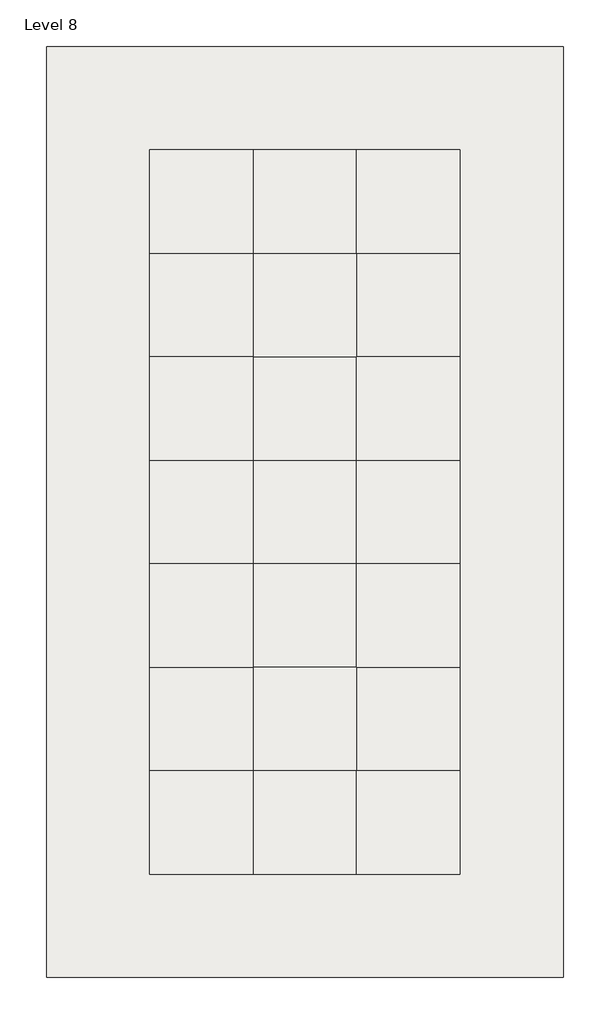
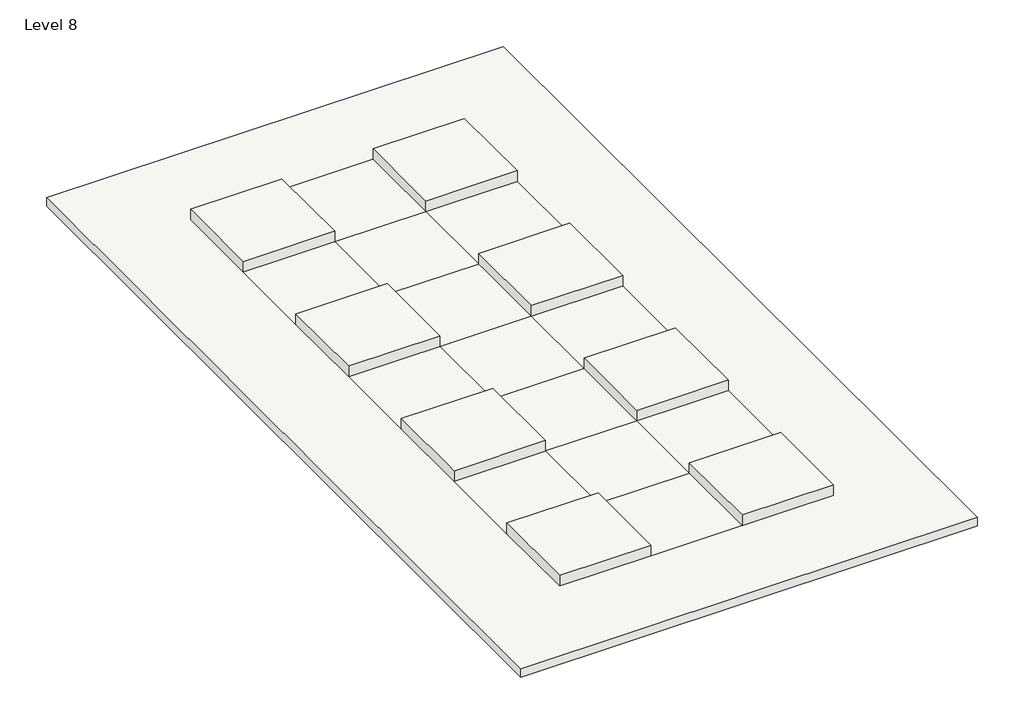
# One storey: 9 roofs.
"""IFC4 building model written with IfcOpenShell, lengths in millimetres."""

import ifcopenshell
import ifcopenshell.guid

model = None  # the IFC model being written
_history = None  # IfcOwnerHistory: only IFC2X3 demands one
_inside = {}  # id of a spatial element -> (the spatial element, [elements in it])
_under = {}  # id of a project, library or spatial element -> (it, [spatial elements below it])
_declared = {}  # id of a project -> (the project, [libraries it declares])
_typed = {}  # id of a type object -> (the type object, [elements of that type])
_made_of = {}  # id of a material, layer set ... -> (it, [elements and type objects made of it])


def new_model(schema):
    """Start an empty IFC model of exactly this schema.

    Asked for "IFC4X3", IfcOpenShell would pick the latest addendum, in which some entities
    have other attributes; the version numbers below select the first issue.
    IFC2X3 requires an IfcOwnerHistory on every rooted entity: one is made here for all.
    """
    global model, _history
    if schema == "IFC4X3":
        model = ifcopenshell.file(schema_version=(4, 3, 0, 0))
    else:
        model = ifcopenshell.file(schema=schema)
    _inside.clear()
    _under.clear()
    _declared.clear()
    _typed.clear()
    _made_of.clear()
    _history = None
    if model.schema == "IFC2X3":
        org = make("IfcOrganization", Name="unknown")
        user = make(
            "IfcPersonAndOrganization",
            ThePerson=make("IfcPerson", FamilyName="unknown"),
            TheOrganization=org,
        )
        app = make(
            "IfcApplication",
            ApplicationDeveloper=org,
            Version="unknown",
            ApplicationFullName="unknown",
            ApplicationIdentifier="unknown",
        )
        _history = make(
            "IfcOwnerHistory",
            OwningUser=user,
            OwningApplication=app,
            ChangeAction="ADDED",
            CreationDate=0,
        )
    return model


def make(cls, **values):
    """One entity of the class cls with the attributes given. An attribute that is None is left unset."""
    return model.create_entity(
        cls, **{name: value for name, value in values.items() if value is not None}
    )


def rooted(cls, **values):
    """An entity with a GlobalId (a new one), such as an element, a storey or a relation."""
    return make(cls, GlobalId=ifcopenshell.guid.new(), OwnerHistory=_history, **values)


def si_unit(unit_type, name, prefix=None):
    """IfcSIUnit, for example si_unit("LENGTHUNIT", "METRE", prefix="MILLI")."""
    return make("IfcSIUnit", UnitType=unit_type, Prefix=prefix, Name=name)


def assignment(units):
    """IfcUnitAssignment: the units of a project."""
    return None if units is None else make("IfcUnitAssignment", Units=units)


def point(xyz):
    """IfcCartesianPoint."""
    return None if xyz is None else make("IfcCartesianPoint", Coordinates=xyz)


def direction(xyz):
    """IfcDirection."""
    return None if xyz is None else make("IfcDirection", DirectionRatios=xyz)


def frame(location, z_axis=None, x_axis=None):
    """IfcAxis2Placement3D, a coordinate frame: its origin and axes. An axis left out is left unset."""
    return make(
        "IfcAxis2Placement3D",
        Location=point(location),
        Axis=direction(z_axis),
        RefDirection=direction(x_axis),
    )


def origin():
    """The frame at (0, 0, 0) with its axes left unset."""
    return frame((0.0, 0.0, 0.0))


def place(relative_to, where):
    """IfcLocalPlacement: puts the frame where relative to a parent placement (None: the world)."""
    return make(
        "IfcLocalPlacement", PlacementRelTo=relative_to, RelativePlacement=where
    )


def context(
    kind, dimensions, precision=None, world=None, true_north=None, identifier=None
):
    """IfcGeometricRepresentationContext, for example the 3D "Model" context."""
    return make(
        "IfcGeometricRepresentationContext",
        ContextIdentifier=identifier,
        ContextType=kind,
        CoordinateSpaceDimension=dimensions,
        Precision=precision,
        WorldCoordinateSystem=world,
        TrueNorth=true_north,
    )


def project(units=None, contexts=None):
    """IfcProject with its units and contexts."""
    return rooted(
        "IfcProject",
        Name="project",
        RepresentationContexts=contexts,
        UnitsInContext=assignment(units),
    )


def spatial(cls, under=None, at=None, **own):
    """A site, building, storey or space (cls), placed at a placement, below another one or the project."""
    s = rooted(cls, ObjectPlacement=at, **own)
    if under is not None:
        _under.setdefault(under.id(), (under, []))[1].append(s)
    return s


def faces_of(points, faces, orient=None, outer=None):
    """IfcFace entities. A face is a list of loops; a loop is a list of indices into points, from 0.

    orient and outer hold one flag for each loop. By default every Orientation is true, the
    first loop of a face is its IfcFaceOuterBound and the others are IfcFaceBound.
    """
    made = []
    for i, loops in enumerate(faces):
        bounds = []
        for j, loop in enumerate(loops):
            is_outer = j == 0 if outer is None else outer[i][j]
            bounds.append(
                make(
                    "IfcFaceOuterBound" if is_outer else "IfcFaceBound",
                    Bound=make("IfcPolyLoop", Polygon=[points[k] for k in loop]),
                    Orientation=True if orient is None else orient[i][j],
                )
            )
        made.append(make("IfcFace", Bounds=bounds))
    return made


def faceted_brep(points, faces, orient=None, outer=None, voids=None):
    """IfcFacetedBrep: a solid bounded by flat faces; with voids (closed shells), ...WithVoids."""
    shared = [point(p) for p in points]
    hull = make("IfcClosedShell", CfsFaces=faces_of(shared, faces, orient, outer))
    if voids is None:
        return make("IfcFacetedBrep", Outer=hull)
    return make(
        "IfcFacetedBrepWithVoids",
        Outer=hull,
        Voids=[
            make(cls, CfsFaces=faces_of(shared, fs, o, b)) for cls, fs, o, b in voids
        ],
    )


def shape(context_of_items, identifier, shape_type, items):
    """IfcShapeRepresentation: the items that make up one representation, for example the "Body"."""
    return make(
        "IfcShapeRepresentation",
        ContextOfItems=context_of_items,
        RepresentationIdentifier=identifier,
        RepresentationType=shape_type,
        Items=items,
    )


def made_of(thing, what):
    """Note that an element or type object is made of a material, layer set ...; save() writes the relation."""
    if what is not None:
        _made_of.setdefault(what.id(), (what, []))[1].append(thing)
    return thing


def element(
    cls,
    number,
    at=None,
    inside=None,
    cuts=None,
    type_object=None,
    material=None,
    context=None,
    identifier="Body",
    shape_type=None,
    held_by="IfcProductDefinitionShape",
    body=None,
    shapes=None,
    **own,
):
    """One element of the class cls, such as IfcWall. Its Tag is "e" and its number.

    at: its placement. inside: the storey or other place that contains it. cuts: it is an
    opening in that element (IfcRelVoidsElement). A single representation is given by context,
    identifier, shape_type and body (its items); several are given by shapes. held_by: the class
    of the entity that holds the representations. save() writes the other relations.
    """
    e = rooted(cls, Tag="e%d" % number, ObjectPlacement=at, **own)
    if body is not None:
        shapes = [shape(context, identifier, shape_type, body)]
    if shapes is not None:
        e.Representation = make(held_by, Representations=shapes)
    if inside is not None:
        _inside.setdefault(inside.id(), (inside, []))[1].append(e)
    if cuts is not None:
        rooted(
            "IfcRelVoidsElement", RelatingBuildingElement=cuts, RelatedOpeningElement=e
        )
    if type_object is not None:
        _typed.setdefault(type_object.id(), (type_object, []))[1].append(e)
    return made_of(e, material)


def aggregate(whole, parts):
    """IfcRelAggregates: a whole, such as a stair, and the parts it consists of."""
    return rooted("IfcRelAggregates", RelatingObject=whole, RelatedObjects=parts)


def save(model, path):
    """Write the relations noted so far, then the file.

    IfcRelAggregates (storeys below a building ...), IfcRelContainedInSpatialStructure (elements
    in a storey), IfcRelDefinesByType, IfcRelAssociatesMaterial and IfcRelDeclares: one each for
    every whole, place, type object, material and project.
    """
    for whole, parts in _under.values():
        aggregate(whole, parts)
    for where, things in _inside.values():
        rooted(
            "IfcRelContainedInSpatialStructure",
            RelatedElements=things,
            RelatingStructure=where,
        )
    for kind, things in _typed.values():
        rooted("IfcRelDefinesByType", RelatedObjects=things, RelatingType=kind)
    for what, things in _made_of.values():
        rooted("IfcRelAssociatesMaterial", RelatedObjects=things, RelatingMaterial=what)
    for by, libraries in _declared.values():
        rooted("IfcRelDeclares", RelatingContext=by, RelatedDefinitions=libraries)
    model.write(path)


model = new_model("IFC4")

# Units and contexts
model_context = context("Model", 3, world=origin())
ifc_project = project(units=[si_unit("LENGTHUNIT", "METRE", prefix="MILLI")], contexts=[model_context])

# Site, building, storey
site = spatial("IfcSite", under=ifc_project)
building = spatial("IfcBuilding", under=site)
storey = spatial("IfcBuildingStorey", under=building, Name="Level 8", Elevation=32000.0)

# Roofs
placement = place(None, origin())
element("IfcRoof", 1, ObjectType="Bauder_RoofCoveringSystem_ExtensiveGreenRoofSystem_WildflowerBlanket", at=placement, inside=storey, context=model_context, shape_type="Brep", body=[
    faceted_brep([(-674.7340554, 1676.2074539, 32000.0), (1325.2659446, 1676.2074539, 32000.0), (1325.2659446, -323.7925461, 32000.0), (-674.7340554, -323.7925461, 32000.0), (1325.2659446, 1676.2074539, 32445.0), (-674.7340554, 1676.2074539, 32445.0), (-674.7340554, -323.7925461, 32445.0), (1325.2659446, -323.7925461, 32445.0), (1325.2659446, 1676.2074539, 32200.0), (-674.7340554, 1676.2074539, 32200.0), (-674.7340554, -323.7925461, 32200.0), (1325.2659446, -323.7925461, 32200.0)], [[[0, 1, 2, 3]], [[4, 5, 6, 7]], [[5, 4, 8, 1, 0, 9]], [[6, 5, 9, 0, 3, 10]], [[7, 6, 10, 3, 2, 11]], [[4, 7, 11, 2, 1, 8]]]),
])
element("IfcRoof", 2, ObjectType="Bauder_RoofCoveringSystem_ExtensiveGreenRoofSystem_WildflowerBlanket", at=placement, inside=storey, context=model_context, shape_type="Brep", body=[
    faceted_brep([(3325.2659446, 1676.2074539, 32000.0), (5325.2659446, 1676.2074539, 32000.0), (5325.2659446, -323.7925461, 32000.0), (3325.2659446, -323.7925461, 32000.0), (5325.2659446, 1676.2074539, 32445.0), (3325.2659446, 1676.2074539, 32445.0), (3325.2659446, -323.7925461, 32445.0), (5325.2659446, -323.7925461, 32445.0), (5325.2659446, 1676.2074539, 32200.0), (3325.2659446, 1676.2074539, 32200.0), (3325.2659446, -323.7925461, 32200.0), (5325.2659446, -323.7925461, 32200.0)], [[[0, 1, 2, 3]], [[4, 5, 6, 7]], [[5, 4, 8, 1, 0, 9]], [[6, 5, 9, 0, 3, 10]], [[7, 6, 10, 3, 2, 11]], [[4, 7, 11, 2, 1, 8]]]),
])
element("IfcRoof", 3, ObjectType="Bauder_RoofCoveringSystem_ExtensiveGreenRoofSystem_WildflowerBlanket", at=placement, inside=storey, context=model_context, shape_type="Brep", body=[
    faceted_brep([(3325.2659446, -2323.7925461, 32000.0), (5325.2659446, -2323.7925461, 32000.0), (5325.2659446, -4323.7925461, 32000.0), (3325.2659446, -4323.7925461, 32000.0), (5325.2659446, -2323.7925461, 32445.0), (3325.2659446, -2323.7925461, 32445.0), (3325.2659446, -4323.7925461, 32445.0), (5325.2659446, -4323.7925461, 32445.0), (5325.2659446, -2323.7925461, 32200.0), (3325.2659446, -2323.7925461, 32200.0), (3325.2659446, -4323.7925461, 32200.0), (5325.2659446, -4323.7925461, 32200.0)], [[[0, 1, 2, 3]], [[4, 5, 6, 7]], [[5, 4, 8, 1, 0, 9]], [[6, 5, 9, 0, 3, 10]], [[7, 6, 10, 3, 2, 11]], [[4, 7, 11, 2, 1, 8]]]),
])
element("IfcRoof", 4, ObjectType="Bauder_RoofCoveringSystem_ExtensiveGreenRoofSystem_WildflowerBlanket", at=placement, inside=storey, context=model_context, shape_type="Brep", body=[
    faceted_brep([(3325.2659446, -6323.7925461, 32000.0), (5325.2659446, -6323.7925461, 32000.0), (5325.2659446, -8323.7925461, 32000.0), (3325.2659446, -8323.7925461, 32000.0), (5325.2659446, -6323.7925461, 32445.0), (3325.2659446, -6323.7925461, 32445.0), (3325.2659446, -8323.7925461, 32445.0), (5325.2659446, -8323.7925461, 32445.0), (3325.2659446, -6323.7925461, 32200.0), (5325.2659446, -6323.7925461, 32200.0), (3325.2659446, -8323.7925461, 32200.0), (5325.2659446, -8323.7925461, 32200.0)], [[[0, 1, 2, 3]], [[4, 5, 6, 7]], [[0, 8, 5, 4, 9, 1]], [[3, 10, 6, 5, 8, 0]], [[2, 11, 7, 6, 10, 3]], [[1, 9, 4, 7, 11, 2]]]),
])
element("IfcRoof", 5, ObjectType="Bauder_RoofCoveringSystem_ExtensiveGreenRoofSystem_WildflowerBlanket", at=placement, inside=storey, context=model_context, shape_type="Brep", body=[
    faceted_brep([(3325.2659446, -10323.7925461, 32000.0), (5325.2659446, -10323.7925461, 32000.0), (5325.2659446, -12323.7925461, 32000.0), (3325.2659446, -12323.7925461, 32000.0), (5325.2659446, -10323.7925461, 32445.0), (3325.2659446, -10323.7925461, 32445.0), (3325.2659446, -12323.7925461, 32445.0), (5325.2659446, -12323.7925461, 32445.0), (3325.2659446, -10323.7925461, 32200.0), (5325.2659446, -10323.7925461, 32200.0), (3325.2659446, -12323.7925461, 32200.0), (5325.2659446, -12323.7925461, 32200.0)], [[[0, 1, 2, 3]], [[4, 5, 6, 7]], [[0, 8, 5, 4, 9, 1]], [[3, 10, 6, 5, 8, 0]], [[2, 11, 7, 6, 10, 3]], [[1, 9, 4, 7, 11, 2]]]),
])
element("IfcRoof", 6, ObjectType="Bauder_RoofCoveringSystem_ExtensiveGreenRoofSystem_WildflowerBlanket", at=placement, inside=storey, context=model_context, shape_type="Brep", body=[
    faceted_brep([(-674.7340554, -10323.7925461, 32000.0), (1325.2659446, -10323.7925461, 32000.0), (1325.2659446, -12323.7925461, 32000.0), (-674.7340554, -12323.7925461, 32000.0), (1325.2659446, -10323.7925461, 32445.0), (-674.7340554, -10323.7925461, 32445.0), (-674.7340554, -12323.7925461, 32445.0), (1325.2659446, -12323.7925461, 32445.0), (1325.2659446, -10323.7925461, 32200.0), (-674.7340554, -10323.7925461, 32200.0), (-674.7340554, -12323.7925461, 32200.0), (1325.2659446, -12323.7925461, 32200.0)], [[[0, 1, 2, 3]], [[4, 5, 6, 7]], [[5, 4, 8, 1, 0, 9]], [[6, 5, 9, 0, 3, 10]], [[7, 6, 10, 3, 2, 11]], [[4, 7, 11, 2, 1, 8]]]),
])
element("IfcRoof", 7, ObjectType="Bauder_RoofCoveringSystem_ExtensiveGreenRoofSystem_WildflowerBlanket", at=placement, inside=storey, context=model_context, shape_type="Brep", body=[
    faceted_brep([(-674.7340554, -6323.7925461, 32000.0), (1325.2659446, -6323.7925461, 32000.0), (1325.2659446, -8323.7925461, 32000.0), (-674.7340554, -8323.7925461, 32000.0), (1325.2659446, -6323.7925461, 32445.0), (-674.7340554, -6323.7925461, 32445.0), (-674.7340554, -8323.7925461, 32445.0), (1325.2659446, -8323.7925461, 32445.0), (1325.2659446, -6323.7925461, 32200.0), (-674.7340554, -6323.7925461, 32200.0), (-674.7340554, -8323.7925461, 32200.0), (1325.2659446, -8323.7925461, 32200.0)], [[[0, 1, 2, 3]], [[4, 5, 6, 7]], [[5, 4, 8, 1, 0, 9]], [[6, 5, 9, 0, 3, 10]], [[7, 6, 10, 3, 2, 11]], [[4, 7, 11, 2, 1, 8]]]),
])
element("IfcRoof", 8, ObjectType="Bauder_RoofCoveringSystem_ExtensiveGreenRoofSystem_WildflowerBlanket", at=placement, inside=storey, context=model_context, shape_type="Brep", body=[
    faceted_brep([(-674.7340554, -2323.7925461, 32000.0), (1325.2659446, -2323.7925461, 32000.0), (1325.2659446, -4323.7925461, 32000.0), (-674.7340554, -4323.7925461, 32000.0), (1325.2659446, -2323.7925461, 32445.0), (-674.7340554, -2323.7925461, 32445.0), (-674.7340554, -4323.7925461, 32445.0), (1325.2659446, -4323.7925461, 32445.0), (1325.2659446, -2323.7925461, 32200.0), (-674.7340554, -2323.7925461, 32200.0), (-674.7340554, -4323.7925461, 32200.0), (1325.2659446, -4323.7925461, 32200.0)], [[[0, 1, 2, 3]], [[4, 5, 6, 7]], [[5, 4, 8, 1, 0, 9]], [[6, 5, 9, 0, 3, 10]], [[7, 6, 10, 3, 2, 11]], [[4, 7, 11, 2, 1, 8]]]),
])
element("IfcRoof", 9, ObjectType="Roof_Concrete-200mm", at=placement, inside=storey, context=model_context, shape_type="Brep", body=[
    faceted_brep([(-2674.7340554, -14323.7925461, 32200.0), (-2674.7340554, -14323.7925461, 32000.0), (7325.2659446, -14323.7925461, 32000.0), (7325.2659446, -14323.7925461, 32200.0), (-2674.7340554, 3676.2074539, 32200.0), (-2674.7340554, 3676.2074539, 32000.0), (7325.2659446, 3676.2074539, 32200.0), (7325.2659446, 3676.2074539, 32000.0), (3325.2659446, 1676.2074539, 32200.0), (1325.2659446, 1676.2074539, 32200.0), (1325.2659446, -323.7925461, 32200.0), (3325.2659446, -323.7925461, 32200.0), (1325.2659446, 1676.2074539, 32000.0), (3325.2659446, 1676.2074539, 32000.0), (3325.2659446, -323.7925461, 32000.0), (1325.2659446, -323.7925461, 32000.0), (1325.2659446, -2323.7925461, 32200.0), (-674.7340554, -323.7925461, 32200.0), (-674.7340554, -2323.7925461, 32200.0), (3325.2659446, -2323.7925461, 32200.0), (5325.2659446, -2323.7925461, 32200.0), (5325.2659446, -323.7925461, 32200.0), (-674.7340554, -2323.7925461, 32000.0), (-674.7340554, -323.7925461, 32000.0), (1325.2659446, -2323.7925461, 32000.0), (3325.2659446, -2323.7925461, 32000.0), (5325.2659446, -323.7925461, 32000.0), (5325.2659446, -2323.7925461, 32000.0), (1325.2659446, -4323.7925461, 32200.0), (3325.2659446, -4323.7925461, 32200.0), (3325.2659446, -4323.7925461, 32000.0), (1325.2659446, -4323.7925461, 32000.0), (1325.2659446, -6323.7925461, 32200.0), (-674.7340554, -4323.7925461, 32200.0), (-674.7340554, -6323.7925461, 32200.0), (5325.2659446, -6323.7925461, 32200.0), (5325.2659446, -4323.7925461, 32200.0), (3325.2659446, -6323.7925461, 32200.0), (-674.7340554, -6323.7925461, 32000.0), (-674.7340554, -4323.7925461, 32000.0), (1325.2659446, -6323.7925461, 32000.0), (3325.2659446, -6323.7925461, 32000.0), (5325.2659446, -4323.7925461, 32000.0), (5325.2659446, -6323.7925461, 32000.0), (1325.2659446, -12323.7925461, 32200.0), (3325.2659446, -12323.7925461, 32200.0), (3325.2659446, -10323.7925461, 32200.0), (1325.2659446, -10323.7925461, 32200.0), (3325.2659446, -12323.7925461, 32000.0), (1325.2659446, -12323.7925461, 32000.0), (1325.2659446, -10323.7925461, 32000.0), (3325.2659446, -10323.7925461, 32000.0), (1325.2659446, -8323.7925461, 32200.0), (-674.7340554, -8323.7925461, 32200.0), (-674.7340554, -10323.7925461, 32200.0), (3325.2659446, -8323.7925461, 32200.0), (5325.2659446, -10323.7925461, 32200.0), (5325.2659446, -8323.7925461, 32200.0), (-674.7340554, -10323.7925461, 32000.0), (-674.7340554, -8323.7925461, 32000.0), (1325.2659446, -8323.7925461, 32000.0), (3325.2659446, -8323.7925461, 32000.0), (5325.2659446, -8323.7925461, 32000.0), (5325.2659446, -10323.7925461, 32000.0), (-674.7340554, 1676.2074539, 32000.0), (-674.7340554, 1676.2074539, 32200.0), (5325.2659446, 1676.2074539, 32200.0), (5325.2659446, 1676.2074539, 32000.0), (5325.2659446, -12323.7925461, 32000.0), (5325.2659446, -12323.7925461, 32200.0), (-674.7340554, -12323.7925461, 32000.0), (-674.7340554, -12323.7925461, 32200.0)], [[[0, 1, 2, 3]], [[1, 0, 4, 5]], [[6, 7, 5, 4]], [[3, 2, 7, 6]], [[8, 9, 10, 11]], [[12, 13, 14, 15]], [[16, 10, 17, 18]], [[11, 10, 16, 19]], [[20, 21, 11, 19]], [[22, 23, 15, 24]], [[15, 14, 25, 24]], [[25, 14, 26, 27]], [[19, 16, 28, 29]], [[24, 25, 30, 31]], [[32, 28, 33, 34]], [[35, 36, 29, 37]], [[38, 39, 31, 40]], [[41, 30, 42, 43]], [[44, 45, 46, 47]], [[48, 49, 50, 51]], [[47, 52, 53, 54]], [[47, 46, 55, 52]], [[56, 57, 55, 46]], [[58, 59, 60, 50]], [[51, 50, 60, 61]], [[51, 61, 62, 63]], [[52, 55, 37, 32]], [[29, 28, 32, 37]], [[61, 60, 40, 41]], [[31, 30, 41, 40]], [[9, 12, 15, 10]], [[10, 15, 23, 17]], [[17, 23, 64, 65]], [[12, 9, 65, 64]], [[66, 67, 26, 21]], [[21, 26, 14, 11]], [[11, 14, 13, 8]], [[67, 66, 8, 13]], [[20, 27, 42, 36]], [[36, 42, 30, 29]], [[29, 30, 25, 19]], [[27, 20, 19, 25]], [[16, 24, 31, 28]], [[28, 31, 39, 33]], [[33, 39, 22, 18]], [[24, 16, 18, 22]], [[32, 40, 60, 52]], [[52, 60, 59, 53]], [[53, 59, 38, 34]], [[40, 32, 34, 38]], [[35, 43, 62, 57]], [[57, 62, 61, 55]], [[55, 61, 41, 37]], [[43, 35, 37, 41]], [[56, 63, 68, 69]], [[69, 68, 48, 45]], [[45, 48, 51, 46]], [[63, 56, 46, 51]], [[47, 50, 49, 44]], [[44, 49, 70, 71]], [[71, 70, 58, 54]], [[50, 47, 54, 58]], [[4, 0, 3, 6], [9, 8, 66, 21, 20, 36, 35, 57, 56, 69, 45, 44, 71, 54, 53, 34, 33, 18, 17, 65]], [[7, 2, 1, 5], [13, 12, 64, 23, 22, 39, 38, 59, 58, 70, 49, 48, 68, 63, 62, 43, 42, 27, 26, 67]]]),
])

save(model, "model.ifc")

# Revit data of these elements
# Type "Bauder_RoofCoveringSystem_ExtensiveGreenRoofSystem_WildflowerBlanket"
#   Keynote = "Q37"
#   Type IFC Predefined Type = "FLAT_ROOF"
#   Export Type to IFC As = "IfcRoofType"
#   Model = "Bauder Biodiverse Wildflower Blanket - Extensive Green Roof System"
#   Manufacturer = "Bauder Ltd"
#   Type Comments = "Wildflower Blanket"
#   URL = "https://www.bauder.co.uk/"
#   Description = "Bauder Biodiverse GreenRoof system incorporating WB 25 mm UK Native Species Wildflower Blanket with Biodiverse Substrate, Filter Fleece, DSE40 Polyethylene Drainage and Protection Layer, and FSM600 Polyester-Polypropylene fibre protection mat."
#   Assembly Code = "B3010"
#   NBSDescription = "Extensive green roof system"
#   NBSReference = "45-40-47/130"
#   BIMObjectName = "Bauder_RoofCoveringSystem_ExtensiveGreenRoofSystem_WildflowerBlanket"
#   AccessibilityPerformance = "n/a"
#   CodePerformance = "n/a"
#   Color = "n/a"
#   Constituents = "n/a"
#   DurationUnit = "Year"
#   ExpectedLife = "n/a"
#   Features = "This BIM Object must be supported by a project specific specification from Bauder, incorporating system build-up, detail design and performance calculations if a full Bauder system guarantee is required. Please contact your local Bauder Representative or technical@bauder.co.uk"
#   Finish = "n/a"
#   Grade = "n/a"
#   Material = "n/a"
#   ModelReference = "Bauder Biodiverse Wildflower Blanket - Extensive Green Roof System"
#   Name = "RoofCoveringSystem_Bauder_ExtensiveGreenRoofSystem"
#   ReplacementCost = "n/a"
#   Shape = "n/a"
#   Size = "n/a"
#   SustainabilityPerformance = "Bauder Germany ISO14001: Certificate No.: 70499/03-15 e, Bauder UK ISO14001:Certificate No. 19ACM6595R, EN1271, BREEAM Credits Available"
#   WarrantyDescription = "Guarantee options could include ‘Product’, ‘Product and Workmanship’ and ‘Product, Workmanship and Design’ Guarantees. All guarantees available for this system are subject to the works being carried out in accordance with the Bauder specification and being installed by a Bauder Approved installer. For full details and further information regarding guarantees and alternative systems please contact your local Bauder Representative or technical@bauder.co.uk"
#   WarrantyDurationLabor = "n/a"
#   WarrantyDurationParts = "n/a"
#   WarrantyDurationUnit = "Year"
#   WarrantyGuarantorLabor = "n/a"
#   WarrantyGuarantorParts = "technical@bauder.co.uk"
#   Certification = "Comply with GRO Green Roof Code of Practice and FLL Standards"
#   EdgeRestraints = "Perforated edge trim where required, refer to Bauder Project Specific Specification"
#   MoistureControlDrainageAncillaries = "n/a"
#   MoistureControlDrainageLayer = "Bauder DSE40 40 mm Polyethylene Drainage and Protection Layer"
#   MoistureControlFilterMembrane = "Bauder Filter Fleece 1 mm Polypropylene Filter Fleece"
#   MoistureControlMoistureRetentionMat = "Polypropylene mesh bonded to a moisture permeable base carrier sheet integral to the Blanket"
#   PlantingSystemsAntierosionMat = "Jute Net where exposed, refer to Bauder Project Specific Specification"
#   PlantingSystemsPlantingMedium = "Bauder Biodiverse Substrate Recycled crushed brick, expanded clay shale and composted pine bark"
#   PlantingSystemsVegetation = "Bauder WB 25 mm UK Native Species Wildflower Blanket"
#   PlantingSystemsVegetationBarrier = "20-40 mm Rounded-Washed Stones, refer to Bauder Project Specific Specification"
#   ProjectSpecificationAndDesign = "This BIM Object must be supported by a project specific specification from Bauder, incorporating system build-up, detail design and performance calculations if a full Bauder system warranty is required. Please contact your local Bauder Representative or technical@bauder.co.uk"
#   ProtectionProtectionLayer = "Bauder FSM600 4 mm Polyester-Polypropylene fibre protection mat"
#   ProtectionRootBarrier = "As per project specific Bauder Specification"
#   ProtectionSeparationLayer = "n/a"
#   SystemManufacturer = "Bauder Ltd"
#   WarrantyConsiderations = "All guarantees available for this system are subject to the works being carried out in accordance with the Bauder specification and being installed by a Bauder Approved installer. For full details and further information regarding guarantees and alternative systems please contact your local Bauder Representative or technical@bauder.co.uk"
#   Update = "1900-12-31T23:59:59"
#   Documentation = "https://www.bauder.co.uk/technical-centre/technical-literature/system-brochures"
#   DocumentReference = "http://www.bauder.co.uk/"
#   IfcExportAs = "IfcRoofType"
#   IfcExportType = "FLAT_ROOF"
#   MethodOfMesurement = "n/a"
#   Process = "Replacement at service life intervals"
#   FireRating = "n/a"
#   _Author = "AM"
#   _AuthorizedBy = "bimstore"
#   _CreatedBy = "technical@bauder.co.uk"
#   _DistributedBy = "www.bimstore.co"
#   AssetType = "Fixed"
#   ClassificationName = "Uniclass2015"
#   ClassificationValue = "Ss_45_40_47_09"
#   CreatedBy = "technical@bauder.co.uk"
#   CreatedOn = "2023-02-10 T00:00:00"
#   DocumentationCertificates = "n/a"
#   DocumentationInstallationGuide = "https://www.bauder.co.uk/technical-centre"
#   DocumentationLiterature = "https://www.bauder.co.uk/technical-centre"
#   DocumentationMaintenance = "https://www.bauder.co.uk/technical-centre/maintenance-advice"
#   DocumentationTechnical = "https://www.bauder.co.uk/green-roofs/extensive-green-roofs/biodiverse-or-brown-roofs/wildflower-blanket"
#   ManufacturerName = "Bauder Ltd"
#   ModelNumber = "0905_WB-BioS-FF-D4-F6"
#   ProductionYear = "2017"
#   ReferencedStandard = "n/a"
#   SpareParts = "n/a"
#   TypeName = "Wildflower Blanket"
#   NBSNote = "n/a"
#   NBSObjectName = "Bauder - Extensive green roof system"
#   NBSOfficeMasterTag = "n/a"
#   Ballast = "n/a"
#   CarrierMembraneFixing = "n/a"
#   CarrierMembraneType = "n/a"
#   FillToPerimeterUpstands = "n/a"
#   FilterLayer = "n/a"
#   InsulationFixing = "n/a"
#   InsulationType = "n/a"
#   LiquidAppliedWaterproofCoatingReinforcement = "n/a"
#   LiquidAppliedWaterproofCoatingSurfaceTreatment = "n/a"
#   LiquidAppliedWaterproofCoatingType = "n/a"
#   PreparationExistingSubstrates = "n/a"
#   PreparationHorizontalWork = "n/a"
#   PreparationSkirtingsAndVerticalWork = "n/a"
#   ProtectionLayer = "n/a"
#   SystemAccessories = "n/a"
#   WaterproofCoveringFirstLayerAttachment = "n/a"
#   WaterproofCoveringFirstLayerType = "n/a"
#   WaterproofCoveringIntermediateLayerAttachment = "n/a"
#   WaterproofCoveringIntermediateLayerType = "n/a"
#   WaterproofCoveringTopLayerAttachment = "n/a"
#   InsulationAttachment = "n/a"
#   IsolatingLayer = "n/a"
#   CarrierMembraneAttachment = "n/a"
#   LiquidAppliedWaterproofCoatingWearingCourse = "n/a"
#   VapourControlLayer = "n/a"
#   VapourControlLayerAttachment_Bauder = "n/a"
#   WaterproofCoveringJoints = "n/a"
#   WaterproofCoveringType = "n/a"
#   SeparatingLayer = "n/a"
#   WaterproofCoveringAccessories = "Yes"
#   WaterproofCoveringAttachment = "n/a"
#   UpperProtectionLayer = "n/a"
#   LowerProtectionLayer = "n/a"
#   WaterproofCoveringTopLayerType = "n/a"
#   DetailWorkAncillaryItems = "Detail as per project specific Bauder Specification"
#   DetailWorkCoverStrips = "Detail as per project specific Bauder Specification"
#   DetailWorkFlashings = "Detail as per project specific Bauder Specification"
#   DetailWorkSkirtingsAndUpstands = "Detail as per project specific Bauder Specification"
#   DetailWorkWeltedDrips = "Detail as per project specific Bauder Specification"
#   OverlayFixing = "n/a"
#   OverlayType = "n/a"
#   SurfaceProtection = "n/a"
#   VapourControlLayerAttachment = "n/a"
#   VapourControlLayerType = "n/a"
#   Cost = 0
#   NominalHeight = 0 mm
#   NominalLength = 0 mm
#   TotalArea = 0 m²
#   NominalDepth = 0 mm
#   IsExternal = yes
#   _BimSpecGuid = 0
#   _BSBibleVersion = 16
#   _CurrentRevision = 4
#   Layers, outside or top first: 100 mm "Bauder_Vegetation_BauderGREEN-WB-Wildflower-Blanket" (function 5); 100 mm "Bauder_ExtensiveSubstrate_BauderGREEN-SUB-BM-UK" (function 2); 1 mm "Bauder_FilterFleece_BauderGREEN-FV-125-100" (function 3); 40 mm "Bauder_DrainageBoard_BauderGREEN-DSE-40" (function 3); 4 mm "Bauder_ProtectionMat_BauderGREEN-FSM-600" (function 3); 200 mm "Concrete" (function 1)
# Type "Roof_Concrete-200mm"
#   Layers, outside or top first: 200 mm "Concrete" (function 1)
# Elements 1, 2, 3, 4, 5, 6, 7, 8 (IfcRoof, "Bauder_RoofCoveringSystem_ExtensiveGreenRoofSystem_WildflowerBlanket")
#   built-in parameter 1001705 = 106.447 (stored number, unit not read)
#   built-in parameter 1001710 = 33615
#   Phase Created = New Construction
#   Materials on its faces: "Concrete", "Bauder_Vegetation_BauderGREEN-WB-Wildflower-Blanket"
# Element 9 (IfcRoof, "Roof_Concrete-200mm")
#   built-in parameter 1001710 = 33615
#   Phase Created = New Construction
#   Materials on its faces: "Concrete"
# Materials
#   "Bauder_Vegetation_BauderGREEN-WB-Wildflower-Blanket": class "Unassigned", colour RGB 71 83 38, transparency 0, Mtrl_Author = "AM", Mtrl_AuthorizedBy = "bimstore", Mtrl_DistributedBy = "www.bimstore.co", Mtrl_AccessibilityPerformance = "n/a", Mtrl_AssetIdentifier = "Please record on commissioning", Mtrl_AssetType = "Fixed", Mtrl_BarCode = "Please record on commissioning", Mtrl_ClassificationName = "Uniclass2020", Mtrl_ClassificationValue = "Ss_45_40_47_09", Mtrl_CodePerformance = "n/a", Mtrl_Color = "n/a", Mtrl_Constituents = "n/a", Mtrl_CreatedBy = "technical@bauder.co.uk", Mtrl_CreatedOn = "2023-02-10 T00:00:00", Mtrl_DocumentationCertificates = "https://www.bimstore.co/products/extensive-green-roof-system-wildflower-blanket/document/product-certificates", Mtrl_DocumentationInstallationGuide = "https://www.bimstore.co/products/extensive-green-roof-system-wildflower-blanket/document/installation-guide", Mtrl_DocumentationLiterature = "https://www.bimstore.co/products/extensive-green-roof-system-wildflower-blanket/document/product-literature", Mtrl_DocumentationMaintenance = "https://www.bimstore.co/products/extensive-green-roof-system-wildflower-blanket/document/maintenance-information", Mtrl_DocumentationTechnical = "https://www.bimstore.co/products/extensive-green-roof-system-wildflower-blanket/document/technical-data-sheet", Mtrl_DurationUnit = "Year", Mtrl_Features = "n/a", Mtrl_Finish = "n/a", Mtrl_Grade = "n/a", Mtrl_InstallationDate = "Please record on commissioning", Mtrl_ManufacturerName = "Bauder Ltd", Mtrl_Material = "Substrate and wildflower plants, embedded in a nylon mesh, with a moisture retention fleece", Mtrl_ModelNumber = "BauderGREEN-WB-Wildflower-Blanket", Mtrl_ModelReference = "Vegetation", Mtrl_ProductionYear = "2023", Mtrl_ReferencedStandard = "n/a", Mtrl_Shape = "n/a", Mtrl_Size = "n/a", Mtrl_SpareParts = "n/a", Mtrl_TypeName = "BauderGREEN-WB-Wildflower-Blanket", Mtrl_WarrantyDescription = "As part of Bauder system guarantee, per specification", Mtrl_WarrantyDurationUnit = "Year", Mtrl_WarrantyGuarantorLabor = "technical@bauder.co.uk", Mtrl_WarrantyGuarantorParts = "technical@bauder.co.uk", Mtrl_WarrantyStartDate = "Please record on commissioning", Mtrl_IfcExportAs = "IfcRoofType", Mtrl_IfcExportType = "FLAT_ROOF", Mtrl_BIMObjectName = "Bauder_Vegetation_BauderGREEN-WB-Wildflower-Blanket", Mtrl_NBSDescription = "n/a", Mtrl_NBSNote = "n/a", Mtrl_NBSObjectName = "n/a", Mtrl_NBSOfficeMasterTag = "n/a", Mtrl_NBSReference = "Q37", Mtrl_Ballast = "n/a", Mtrl_CarrierMembraneAttachment = "n/a", Mtrl_CarrierMembraneFixing = "n/a", Mtrl_CarrierMembraneType = "n/a", Mtrl_Certification = "Comply with GRO Green Roof Code of Practice and FLL Standards", Mtrl_DetailWorkAncillaryItems = "Detail as per project specific Bauder Specification", Mtrl_DetailWorkCoverStrips = "Detail as per project specific Bauder Specification", Mtrl_DetailWorkFlashings = "Detail as per project specific Bauder Specification", Mtrl_DetailWorkSkirtingsAndUpstands = "Detail as per project specific Bauder Specification", Mtrl_DetailWorkWeltedDrips = "Detail as per project specific Bauder Specification", Mtrl_EdgeRestraints = "Detail as per project specific Bauder Specification", Mtrl_FillToPerimeterUpstands = "n/a", Mtrl_FilterLayer = "n/a", Mtrl_InsulationAttachment = "As per project specific Bauder Specification", Mtrl_InsulationFixing = "As per project specific Bauder Specification", Mtrl_InsulationType = "As per project specific Bauder Specification", Mtrl_IsolatingLayer = "n/a", Mtrl_LiquidAppliedWaterproofCoatingReinforcement = "As per project specific Bauder Specification", Mtrl_LiquidAppliedWaterproofCoatingSurfaceTreatment = "As per project specific Bauder Specification", Mtrl_LiquidAppliedWaterproofCoatingType = "As per project specific Bauder Specification", Mtrl_LiquidAppliedWaterproofCoatingWearingCourse = "As per project specific Bauder Specification", Mtrl_LowerProtectionLayer = "n/a", Mtrl_MoistureControlDrainageAncillaries = "n/a", Mtrl_MoistureControlDrainageLayer = "n/a", Mtrl_MoistureControlFilterMembrane = "n/a", Mtrl_MoistureControlMoistureRetentionMat = "n/a", Mtrl_OverlayFixing = "n/a", Mtrl_OverlayType = "n/a", Mtrl_PlantingSystemsAntierosionMat = "n/a", Mtrl_PlantingSystemsPlantingMedium = "As per project specific Bauder Specification", Mtrl_PlantingSystemsVegetation = "As per project specific Bauder Specification", Mtrl_PlantingSystemsVegetationBarrier = "As per project specific Bauder Specification", Mtrl_PreparationExistingSubstrates = "n/a", Mtrl_PreparationHorizontalWork = "n/a", Mtrl_PreparationSkirtingsAndVerticalWork = "n/a", Mtrl_ProjectSpecificationAndDesign = "This BIM Object must be supported by a project specific specification from Bauder, incorporating system build-up, detail design and performance calculations if a full Bauder system warranty is required. Please contact your local Bauder Representative or technical@bauder.co.uk", Mtrl_ProtectionLayer = "n/a", Mtrl_ProtectionProtectionLayer = "n/a", Mtrl_ProtectionRootBarrier = "As per project specific Bauder Specification", Mtrl_ProtectionSeparationLayer = "n/a", Mtrl_SeparatingLayer = "n/a", Mtrl_SurfaceProtection = "n/a", Mtrl_SystemAccessories = "n/a", Mtrl_SystemManufacturer = "Bauder Ltd", Mtrl_Update = "1900-12-31 T23:59:59", Mtrl_UpperProtectionLayer = "n/a", Mtrl_VapourControlLayerAttachment = "As per project specific Bauder Specification", Mtrl_VapourControlLayerAttachment_Bauder = "As per project specific Bauder Specification", Mtrl_VapourControlLayerType = "As per project specific Bauder Specification", Mtrl_WarrantyConsiderations = "All guarantees available for this system are subject to the works being carried out in accordance with the Bauder specification and being installed by a Bauder Approved installer. For full details and further information regarding guarantees and alternative systems please contact your local Bauder Representative or technical@bauder.co.uk", Mtrl_WaterproofCoveringAccessories = "As per project specific Bauder Specification", Mtrl_WaterproofCoveringAttachment = "As per project specific Bauder Specification", Mtrl_WaterproofCoveringFirstLayerAttachment = "As per project specific Bauder Specification", Mtrl_WaterproofCoveringFirstLayerType = "As per project specific Bauder Specification", Mtrl_WaterproofCoveringIntermediateLayerAttachment = "As per project specific Bauder Specification", Mtrl_WaterproofCoveringIntermediateLayerType = "As per project specific Bauder Specification", Mtrl_WaterproofCoveringJoints = "As per project specific Bauder Specification", Mtrl_WaterproofCoveringTopLayerAttachment = "As per project specific Bauder Specification", Mtrl_WaterproofCoveringTopLayerType = "As per project specific Bauder Specification", Mtrl_WaterproofCoveringType = "As per project specific Bauder Specification", Cost = 0, Mtrl_ReplacementCost = 0, Mtrl_NominalDepth = 30 mm, Mtrl_NominalHeight = 0 mm, Mtrl_NominalLength = 0 mm, Mtrl_BimSpecGuid = 0, Mtrl_BSBibleVersion = 17, Mtrl_CurrentRevision = 2, Mtrl_ExpectedLife = 0, Mtrl_SerialNumber = 0, Mtrl_WarrantyDurationLabor = 0, Mtrl_WarrantyDurationParts = 0
#   "Bauder_ExtensiveSubstrate_BauderGREEN-SUB-BM-UK": class "Unassigned", colour RGB 255 255 255, transparency 0, Mtrl_Author = "AM", Mtrl_AuthorizedBy = "bimstore", Mtrl_DistributedBy = "www.bimstore.co", Mtrl_AccessibilityPerformance = "n/a", Mtrl_AssetIdentifier = "Please record on commissioning", Mtrl_AssetType = "Fixed", Mtrl_BarCode = "Please record on commissioning", Mtrl_ClassificationName = "Uniclass2019", Mtrl_ClassificationValue = "n/a", Mtrl_CodePerformance = "n/a", Mtrl_Color = "n/a", Mtrl_Constituents = "n/a", Mtrl_CreatedBy = "technical@bauder.co.uk", Mtrl_CreatedOn = "2023-02-10 T00:00:00", Mtrl_DocumentationCertificates = "https://www.bimstore.co/products/extensive-green-roof-system-wildflower-blanket/document/product-certificates", Mtrl_DocumentationInstallationGuide = "https://www.bimstore.co/products/extensive-green-roof-system-wildflower-blanket/document/installation-guide", Mtrl_DocumentationLiterature = "https://www.bimstore.co/products/extensive-green-roof-system-wildflower-blanket/document/product-literature", Mtrl_DocumentationMaintenance = "https://www.bimstore.co/products/extensive-green-roof-system-wildflower-blanket/document/maintenance-information", Mtrl_DocumentationTechnical = "https://www.bimstore.co/products/extensive-green-roof-system-wildflower-blanket/document/technical-data-sheet", Mtrl_DurationUnit = "Year", Mtrl_Features = "n/a", Mtrl_Finish = "n/a", Mtrl_Grade = "n/a", Mtrl_InstallationDate = "Please record on commissioning", Mtrl_ManufacturerName = "Bauder Ltd", Mtrl_Material = "Recycled crushed brick, expanded clay, shale, composted pine bark", Mtrl_ModelNumber = "BauderGREEN-SUB-BM-UK", Mtrl_ModelReference = "Extensive Substrate", Mtrl_ProductionYear = "2023", Mtrl_ReferencedStandard = "n/a", Mtrl_Shape = "n/a", Mtrl_Size = "n/a", Mtrl_SpareParts = "n/a", Mtrl_TypeName = "BauderGREEN-SUB-BM-UK", Mtrl_WarrantyDescription = "As part of Bauder system guarantee, per specification", Mtrl_WarrantyDurationUnit = "Year", Mtrl_WarrantyGuarantorLabor = "technical@bauder.co.uk", Mtrl_WarrantyGuarantorParts = "technical@bauder.co.uk", Mtrl_WarrantyStartDate = "Please record on commissioning", Mtrl_IfcExportAs = "IfcRoofType", Mtrl_IfcExportType = "FLAT_ROOF", Mtrl_BIMObjectName = "Bauder_ExtensiveSubstrate_BauderGREEN-SUB-BM-UK", Mtrl_NBSDescription = "n/a", Mtrl_NBSNote = "n/a", Mtrl_NBSObjectName = "n/a", Mtrl_NBSOfficeMasterTag = "n/a", Mtrl_NBSReference = "Q37", Mtrl_Ballast = "n/a", Mtrl_CarrierMembraneAttachment = "n/a", Mtrl_CarrierMembraneFixing = "n/a", Mtrl_CarrierMembraneType = "n/a", Mtrl_Certification = "Comply with GRO Green Roof Code of Practice and FLL Standards", Mtrl_DetailWorkAncillaryItems = "Detail as per project specific Bauder Specification", Mtrl_DetailWorkCoverStrips = "Detail as per project specific Bauder Specification", Mtrl_DetailWorkFlashings = "Detail as per project specific Bauder Specification", Mtrl_DetailWorkSkirtingsAndUpstands = "Detail as per project specific Bauder Specification", Mtrl_DetailWorkWeltedDrips = "Detail as per project specific Bauder Specification", Mtrl_EdgeRestraints = "Detail as per project specific Bauder Specification", Mtrl_FillToPerimeterUpstands = "n/a", Mtrl_FilterLayer = "n/a", Mtrl_InsulationAttachment = "As per project specific Bauder Specification", Mtrl_InsulationFixing = "As per project specific Bauder Specification", Mtrl_InsulationType = "As per project specific Bauder Specification", Mtrl_IsolatingLayer = "n/a", Mtrl_LiquidAppliedWaterproofCoatingReinforcement = "As per project specific Bauder Specification", Mtrl_LiquidAppliedWaterproofCoatingSurfaceTreatment = "As per project specific Bauder Specification", Mtrl_LiquidAppliedWaterproofCoatingType = "As per project specific Bauder Specification", Mtrl_LiquidAppliedWaterproofCoatingWearingCourse = "As per project specific Bauder Specification", Mtrl_LowerProtectionLayer = "As per project specific Bauder Specification", Mtrl_MoistureControlDrainageAncillaries = "n/a", Mtrl_MoistureControlDrainageLayer = "n/a", Mtrl_MoistureControlFilterMembrane = "n/a", Mtrl_MoistureControlMoistureRetentionMat = "n/a", Mtrl_OverlayFixing = "n/a", Mtrl_OverlayType = "n/a", Mtrl_PlantingSystemsAntierosionMat = "n/a", Mtrl_PlantingSystemsPlantingMedium = "As per project specific Bauder Specification", Mtrl_PlantingSystemsVegetation = "As per project specific Bauder Specification", Mtrl_PlantingSystemsVegetationBarrier = "As per project specific Bauder Specification", Mtrl_PreparationExistingSubstrates = "n/a", Mtrl_PreparationHorizontalWork = "n/a", Mtrl_PreparationSkirtingsAndVerticalWork = "n/a", Mtrl_ProjectSpecificationAndDesign = "This BIM Object must be supported by a project specific specification from Bauder, incorporating system build-up, detail design and performance calculations if a full Bauder system warranty is required. Please contact your local Bauder Representative or technical@bauder.co.uk", Mtrl_ProtectionLayer = "n/a", Mtrl_ProtectionProtectionLayer = "n/a", Mtrl_ProtectionRootBarrier = "As per project specific Bauder Specification", Mtrl_ProtectionSeparationLayer = "n/a", Mtrl_SeparatingLayer = "n/a", Mtrl_SurfaceProtection = "n/a", Mtrl_SystemAccessories = "n/a", Mtrl_SystemManufacturer = "Bauder Ltd", Mtrl_Update = "1900-12-31 T23:59:59", Mtrl_UpperProtectionLayer = "n/a", Mtrl_VapourControlLayerAttachment = "As per project specific Bauder Specification", Mtrl_VapourControlLayerAttachment_Bauder = "As per project specific Bauder Specification", Mtrl_VapourControlLayerType = "As per project specific Bauder Specification", Mtrl_WarrantyConsiderations = "All guarantees available for this system are subject to the works being carried out in accordance with the Bauder specification and being installed by a Bauder Approved installer. For full details and further information regarding guarantees and alternative systems please contact your local Bauder Representative or technical@bauder.co.uk", Mtrl_WaterproofCoveringAccessories = "As per project specific Bauder Specification", Mtrl_WaterproofCoveringAttachment = "As per project specific Bauder Specification", Mtrl_WaterproofCoveringFirstLayerAttachment = "As per project specific Bauder Specification", Mtrl_WaterproofCoveringFirstLayerType = "As per project specific Bauder Specification", Mtrl_WaterproofCoveringIntermediateLayerAttachment = "As per project specific Bauder Specification", Mtrl_WaterproofCoveringIntermediateLayerType = "As per project specific Bauder Specification", Mtrl_WaterproofCoveringJoints = "As per project specific Bauder Specification", Mtrl_WaterproofCoveringTopLayerAttachment = "As per project specific Bauder Specification", Mtrl_WaterproofCoveringTopLayerType = "As per project specific Bauder Specification", Mtrl_WaterproofCoveringType = "As per project specific Bauder Specification", Cost = 0, Mtrl_ReplacementCost = 0, Mtrl_NominalDepth = 100 mm, Mtrl_NominalHeight = 0 mm, Mtrl_NominalLength = 0 mm, Mtrl_BimSpecGuid = 0, Mtrl_BSBibleVersion = 17, Mtrl_CurrentRevision = 2, Mtrl_ExpectedLife = 0, Mtrl_SerialNumber = 0, Mtrl_WarrantyDurationLabor = 0, Mtrl_WarrantyDurationParts = 0
#   "Bauder_FilterFleece_BauderGREEN-FV-125-100": class "Unassigned", colour RGB 255 255 255, transparency 0, Mtrl_Author = "AM", Mtrl_AuthorizedBy = "bimstore", Mtrl_DistributedBy = "www.bimstore.co", Mtrl_AccessibilityPerformance = "n/a", Mtrl_AssetIdentifier = "Please record on commissioning", Mtrl_AssetType = "Fixed", Mtrl_BarCode = "Please record on commissioning", Mtrl_ClassificationName = "Uniclass2015", Mtrl_ClassificationValue = "n/a", Mtrl_CodePerformance = "n/a", Mtrl_Color = "n/a", Mtrl_Constituents = "n/a", Mtrl_CreatedBy = "technical@bauder.co.uk", Mtrl_CreatedOn = "2023-02-10 T00:00:00", Mtrl_DocumentationCertificates = "https://www.bimstore.co/products/extensive-green-roof-system-wildflower-blanket/document/product-certificates", Mtrl_DocumentationInstallationGuide = "https://www.bimstore.co/products/extensive-green-roof-system-wildflower-blanket/document/installation-guide", Mtrl_DocumentationLiterature = "https://www.bimstore.co/products/intensive-green-roof-system/document/product-literature", Mtrl_DocumentationMaintenance = "https://www.bimstore.co/products/extensive-green-roof-system-wildflower-blanket/document/maintenance-information", Mtrl_DocumentationTechnical = "https://www.bimstore.co/products/extensive-green-roof-system-wildflower-blanket/document/technical-data-sheet", Mtrl_DurationUnit = "Year", Mtrl_Features = "n/a", Mtrl_Finish = "n/a", Mtrl_Grade = "n/a", Mtrl_InstallationDate = "Please record on commissioning", Mtrl_ManufacturerName = "Bauder Ltd", Mtrl_Material = "Polypropylene Fleece", Mtrl_ModelNumber = "BauderGREEN-FV-125-100", Mtrl_ModelReference = "Filter Fleece", Mtrl_ProductionYear = "2023", Mtrl_ReferencedStandard = "n/a", Mtrl_Shape = "n/a", Mtrl_Size = "n/a", Mtrl_SpareParts = "n/a", Mtrl_TypeName = "BauderGREEN-FV-125-100", Mtrl_WarrantyDescription = "As part of Bauder system guarantee, per specification", Mtrl_WarrantyDurationUnit = "Year", Mtrl_WarrantyGuarantorLabor = "technical@bauder.co.uk", Mtrl_WarrantyGuarantorParts = "technical@bauder.co.uk", Mtrl_WarrantyStartDate = "Please record on commissioning", Mtrl_IfcExportAs = "IfcRoofType", Mtrl_IfcExportType = "FLAT_ROOF", Mtrl_BIMObjectName = "Bauder_FilterFleece_BauderGREEN-FV-125-100", Mtrl_NBSDescription = "n/a", Mtrl_NBSNote = "n/a", Mtrl_NBSObjectName = "n/a", Mtrl_NBSOfficeMasterTag = "n/a", Mtrl_NBSReference = "Q37", Mtrl_Ballast = "n/a", Mtrl_CarrierMembraneAttachment = "n/a", Mtrl_CarrierMembraneFixing = "n/a", Mtrl_CarrierMembraneType = "n/a", Mtrl_Certification = "Comply with GRO Green Roof Code of Practice and FLL Standards", Mtrl_DetailWorkAncillaryItems = "Detail as per project specific Bauder Specification", Mtrl_DetailWorkCoverStrips = "Detail as per project specific Bauder Specification", Mtrl_DetailWorkFlashings = "Detail as per project specific Bauder Specification", Mtrl_DetailWorkSkirtingsAndUpstands = "Detail as per project specific Bauder Specification", Mtrl_DetailWorkWeltedDrips = "Detail as per project specific Bauder Specification", Mtrl_EdgeRestraints = "Detail as per project specific Bauder Specification", Mtrl_FillToPerimeterUpstands = "n/a", Mtrl_FilterLayer = "n/a", Mtrl_InsulationAttachment = "As per project specific Bauder Specification", Mtrl_InsulationFixing = "As per project specific Bauder Specification", Mtrl_InsulationType = "As per project specific Bauder Specification", Mtrl_IsolatingLayer = "n/a", Mtrl_LiquidAppliedWaterproofCoatingReinforcement = "As per project specific Bauder Specification", Mtrl_LiquidAppliedWaterproofCoatingSurfaceTreatment = "As per project specific Bauder Specification", Mtrl_LiquidAppliedWaterproofCoatingType = "As per project specific Bauder Specification", Mtrl_LiquidAppliedWaterproofCoatingWearingCourse = "As per project specific Bauder Specification", Mtrl_LowerProtectionLayer = "n/a", Mtrl_MoistureControlDrainageAncillaries = "n/a", Mtrl_MoistureControlDrainageLayer = "n/a", Mtrl_MoistureControlFilterMembrane = "n/a", Mtrl_MoistureControlMoistureRetentionMat = "n/a", Mtrl_OverlayFixing = "n/a", Mtrl_OverlayType = "n/a", Mtrl_PlantingSystemsAntierosionMat = "n/a", Mtrl_PlantingSystemsPlantingMedium = "As per project specific Bauder Specification", Mtrl_PlantingSystemsVegetation = "As per project specific Bauder Specification", Mtrl_PlantingSystemsVegetationBarrier = "As per project specific Bauder Specification", Mtrl_PreparationExistingSubstrates = "n/a", Mtrl_PreparationHorizontalWork = "n/a", Mtrl_PreparationSkirtingsAndVerticalWork = "n/a", Mtrl_ProjectSpecificationAndDesign = "This BIM Object must be supported by a project specific specification from Bauder, incorporating system build-up, detail design and performance calculations if a full Bauder system warranty is required. Please contact your local Bauder Representative or technical@bauder.co.uk", Mtrl_ProtectionLayer = "n/a", Mtrl_ProtectionProtectionLayer = "n/a", Mtrl_ProtectionRootBarrier = "As per project specific Bauder Specification", Mtrl_ProtectionSeparationLayer = "n/a", Mtrl_SeparatingLayer = "n/a", Mtrl_SurfaceProtection = "n/a", Mtrl_SystemAccessories = "n/a", Mtrl_SystemManufacturer = "Bauder Ltd", Mtrl_Update = "1900-12-31 T23:59:59", Mtrl_UpperProtectionLayer = "n/a", Mtrl_VapourControlLayerAttachment = "As per project specific Bauder Specification", Mtrl_VapourControlLayerAttachment_Bauder = "As per project specific Bauder Specification", Mtrl_VapourControlLayerType = "As per project specific Bauder Specification", Mtrl_WarrantyConsiderations = "All guarantees available for this system are subject to the works being carried out in accordance with the Bauder specification and being installed by a Bauder Approved installer. For full details and further information regarding guarantees and alternative systems please contact your local Bauder Representative or technical@bauder.co.uk", Mtrl_WaterproofCoveringAccessories = "As per project specific Bauder Specification", Mtrl_WaterproofCoveringAttachment = "As per project specific Bauder Specification", Mtrl_WaterproofCoveringFirstLayerAttachment = "As per project specific Bauder Specification", Mtrl_WaterproofCoveringFirstLayerType = "As per project specific Bauder Specification", Mtrl_WaterproofCoveringIntermediateLayerAttachment = "As per project specific Bauder Specification", Mtrl_WaterproofCoveringIntermediateLayerType = "As per project specific Bauder Specification", Mtrl_WaterproofCoveringJoints = "As per project specific Bauder Specification", Mtrl_WaterproofCoveringTopLayerAttachment = "As per project specific Bauder Specification", Mtrl_WaterproofCoveringTopLayerType = "As per project specific Bauder Specification", Mtrl_WaterproofCoveringType = "As per project specific Bauder Specification", Cost = 0, Mtrl_ReplacementCost = 0, Mtrl_NominalDepth = 1 mm, Mtrl_NominalHeight = 0 mm, Mtrl_NominalLength = 0 mm, Mtrl_BimSpecGuid = 0, Mtrl_BSBibleVersion = 17, Mtrl_CurrentRevision = 2, Mtrl_ExpectedLife = 0, Mtrl_SerialNumber = 0, Mtrl_WarrantyDurationLabor = 0, Mtrl_WarrantyDurationParts = 0
#   "Bauder_DrainageBoard_BauderGREEN-DSE-40": class "Unassigned", colour RGB 255 255 255, transparency 0, Mtrl_Author = "AM", Mtrl_AuthorizedBy = "bimstore", Mtrl_DistributedBy = "www.bimstore.co", Mtrl_AccessibilityPerformance = "n/a", Mtrl_AssetIdentifier = "Please record on commissioning", Mtrl_AssetType = "Fixed", Mtrl_BarCode = "Please record on commissioning", Mtrl_ClassificationName = "Uniclass2015", Mtrl_ClassificationValue = "Pr_65_67_78_72", Mtrl_CodePerformance = "n/a", Mtrl_Color = "n/a", Mtrl_Constituents = "n/a", Mtrl_CreatedBy = "technical@bauder.co.uk", Mtrl_CreatedOn = "2023-02-10 T00:00:00", Mtrl_DocumentationCertificates = "https://www.bimstore.co/products/extensive-green-roof-system-wildflower-blanket/document/product-certificates", Mtrl_DocumentationInstallationGuide = "https://www.bimstore.co/products/extensive-green-roof-system-wildflower-blanket/document/installation-guide", Mtrl_DocumentationLiterature = "https://www.bimstore.co/products/extensive-green-roof-system-wildflower-blanket/document/product-literature", Mtrl_DocumentationMaintenance = "https://www.bimstore.co/products/extensive-green-roof-system-wildflower-blanket/document/maintenance-information", Mtrl_DocumentationTechnical = "https://www.bimstore.co/products/extensive-green-roof-system-wildflower-blanket/document/technical-data-sheet", Mtrl_DurationUnit = "Year", Mtrl_Features = "n/a", Mtrl_Finish = "n/a", Mtrl_Grade = "n/a", Mtrl_InstallationDate = "Please record on commissioning", Mtrl_ManufacturerName = "Bauder Ltd", Mtrl_Material = "Recycled High Density Polyethylene", Mtrl_ModelNumber = "BauderGREEN-DSE-40", Mtrl_ModelReference = "Drainage Board", Mtrl_ProductionYear = "2023", Mtrl_ReferencedStandard = "n/a", Mtrl_Shape = "n/a", Mtrl_Size = "n/a", Mtrl_SpareParts = "n/a", Mtrl_TypeName = "BauderGREEN-DSE-40", Mtrl_WarrantyDescription = "As part of Bauder system guarantee, per specification", Mtrl_WarrantyDurationUnit = "Year", Mtrl_WarrantyGuarantorLabor = "technical@bauder.co.uk", Mtrl_WarrantyGuarantorParts = "technical@bauder.co.uk", Mtrl_WarrantyStartDate = "Please record on commissioning", Mtrl_IfcExportAs = "IfcRoofType", Mtrl_IfcExportType = "FLAT_ROOF", Mtrl_BIMObjectName = "Bauder_DrainageBoard_BauderGREEN-DSE-40", Mtrl_NBSDescription = "n/a", Mtrl_NBSNote = "n/a", Mtrl_NBSObjectName = "n/a", Mtrl_NBSOfficeMasterTag = "n/a", Mtrl_NBSReference = "Q37", Mtrl_Ballast = "n/a", Mtrl_CarrierMembraneAttachment = "n/a", Mtrl_CarrierMembraneFixing = "n/a", Mtrl_CarrierMembraneType = "n/a", Mtrl_Certification = "Comply with GRO Green Roof Code of Practice and FLL Standards", Mtrl_DetailWorkAncillaryItems = "Detail as per project specific Bauder Specification", Mtrl_DetailWorkCoverStrips = "Detail as per project specific Bauder Specification", Mtrl_DetailWorkFlashings = "Detail as per project specific Bauder Specification", Mtrl_DetailWorkSkirtingsAndUpstands = "Detail as per project specific Bauder Specification", Mtrl_DetailWorkWeltedDrips = "Detail as per project specific Bauder Specification", Mtrl_EdgeRestraints = "Detail as per project specific Bauder Specification", Mtrl_FillToPerimeterUpstands = "n/a", Mtrl_FilterLayer = "n/a", Mtrl_InsulationAttachment = "As per project specific Bauder Specification", Mtrl_InsulationFixing = "As per project specific Bauder Specification", Mtrl_InsulationType = "As per project specific Bauder Specification", Mtrl_IsolatingLayer = "n/a", Mtrl_LiquidAppliedWaterproofCoatingReinforcement = "As per project specific Bauder Specification", Mtrl_LiquidAppliedWaterproofCoatingSurfaceTreatment = "As per project specific Bauder Specification", Mtrl_LiquidAppliedWaterproofCoatingType = "As per project specific Bauder Specification", Mtrl_LiquidAppliedWaterproofCoatingWearingCourse = "As per project specific Bauder Specification", Mtrl_LowerProtectionLayer = "n/a", Mtrl_MoistureControlDrainageAncillaries = "n/a", Mtrl_MoistureControlDrainageLayer = "n/a", Mtrl_MoistureControlFilterMembrane = "n/a", Mtrl_MoistureControlMoistureRetentionMat = "n/a", Mtrl_OverlayFixing = "n/a", Mtrl_OverlayType = "n/a", Mtrl_PlantingSystemsAntierosionMat = "n/a", Mtrl_PlantingSystemsPlantingMedium = "As per project specific Bauder Specification", Mtrl_PlantingSystemsVegetation = "As per project specific Bauder Specification", Mtrl_PlantingSystemsVegetationBarrier = "As per project specific Bauder Specification", Mtrl_PreparationExistingSubstrates = "n/a", Mtrl_PreparationHorizontalWork = "n/a", Mtrl_PreparationSkirtingsAndVerticalWork = "n/a", Mtrl_ProjectSpecificationAndDesign = "This BIM Object must be supported by a project specific specification from Bauder, incorporating system build-up, detail design and performance calculations if a full Bauder system warranty is required. Please contact your local Bauder Representative or technical@bauder.co.uk", Mtrl_ProtectionLayer = "n/a", Mtrl_ProtectionProtectionLayer = "n/a", Mtrl_ProtectionRootBarrier = "As per project specific Bauder Specification", Mtrl_ProtectionSeparationLayer = "n/a", Mtrl_SeparatingLayer = "n/a", Mtrl_SurfaceProtection = "n/a", Mtrl_SystemAccessories = "n/a", Mtrl_SystemManufacturer = "Bauder Ltd", Mtrl_Update = "1900-12-31 T23:59:59", Mtrl_UpperProtectionLayer = "n/a", Mtrl_VapourControlLayerAttachment = "As per project specific Bauder Specification", Mtrl_VapourControlLayerAttachment_Bauder = "As per project specific Bauder Specification", Mtrl_VapourControlLayerType = "As per project specific Bauder Specification", Mtrl_WarrantyConsiderations = "All guarantees available for this system are subject to the works being carried out in accordance with the Bauder specification and being installed by a Bauder Approved installer. For full details and further information regarding guarantees and alternative systems please contact your local Bauder Representative or technical@bauder.co.uk", Mtrl_WaterproofCoveringAccessories = "As per project specific Bauder Specification", Mtrl_WaterproofCoveringAttachment = "As per project specific Bauder Specification", Mtrl_WaterproofCoveringFirstLayerAttachment = "As per project specific Bauder Specification", Mtrl_WaterproofCoveringFirstLayerType = "As per project specific Bauder Specification", Mtrl_WaterproofCoveringIntermediateLayerAttachment = "As per project specific Bauder Specification", Mtrl_WaterproofCoveringIntermediateLayerType = "As per project specific Bauder Specification", Mtrl_WaterproofCoveringJoints = "As per project specific Bauder Specification", Mtrl_WaterproofCoveringTopLayerAttachment = "As per project specific Bauder Specification", Mtrl_WaterproofCoveringTopLayerType = "As per project specific Bauder Specification", Mtrl_WaterproofCoveringType = "As per project specific Bauder Specification", Cost = 0, Mtrl_ReplacementCost = 0, Mtrl_NominalDepth = 40 mm, Mtrl_NominalHeight = 0 mm, Mtrl_NominalLength = 0 mm, Mtrl_BimSpecGuid = 0, Mtrl_BSBibleVersion = 17, Mtrl_CurrentRevision = 2, Mtrl_ExpectedLife = 0, Mtrl_SerialNumber = 0, Mtrl_WarrantyDurationLabor = 0, Mtrl_WarrantyDurationParts = 0
